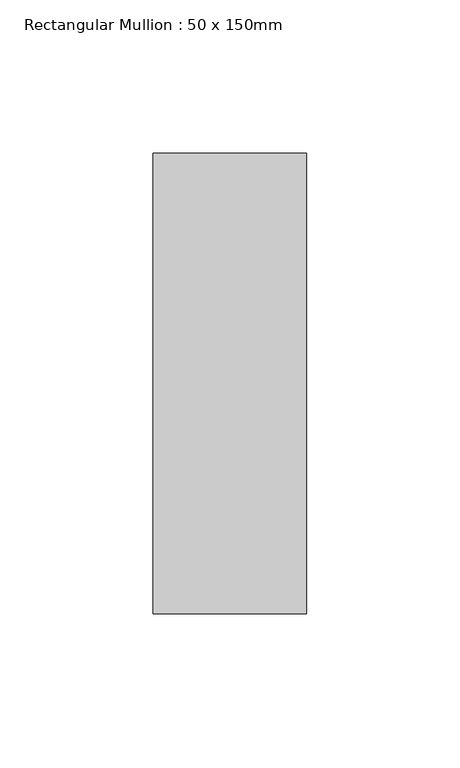
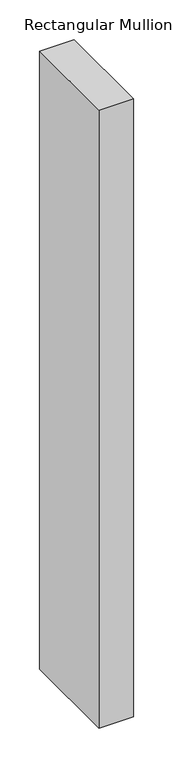
"""IFC4 building model written with IfcOpenShell, lengths in millimetres: member geometry, Rectangular Mullion : 50 x 150mm."""

import ifcopenshell
import ifcopenshell.guid

model = None  # the IFC model being written
_history = None  # IfcOwnerHistory: only IFC2X3 demands one
_inside = {}  # id of a spatial element -> (the spatial element, [elements in it])
_under = {}  # id of a project, library or spatial element -> (it, [spatial elements below it])
_declared = {}  # id of a project -> (the project, [libraries it declares])
_typed = {}  # id of a type object -> (the type object, [elements of that type])
_made_of = {}  # id of a material, layer set ... -> (it, [elements and type objects made of it])


def new_model(schema):
    """Start an empty IFC model of exactly this schema.

    Asked for "IFC4X3", IfcOpenShell would pick the latest addendum, in which some entities
    have other attributes; the version numbers below select the first issue.
    IFC2X3 requires an IfcOwnerHistory on every rooted entity: one is made here for all.
    """
    global model, _history
    if schema == "IFC4X3":
        model = ifcopenshell.file(schema_version=(4, 3, 0, 0))
    else:
        model = ifcopenshell.file(schema=schema)
    _inside.clear()
    _under.clear()
    _declared.clear()
    _typed.clear()
    _made_of.clear()
    _history = None
    if model.schema == "IFC2X3":
        org = make("IfcOrganization", Name="unknown")
        user = make(
            "IfcPersonAndOrganization",
            ThePerson=make("IfcPerson", FamilyName="unknown"),
            TheOrganization=org,
        )
        app = make(
            "IfcApplication",
            ApplicationDeveloper=org,
            Version="unknown",
            ApplicationFullName="unknown",
            ApplicationIdentifier="unknown",
        )
        _history = make(
            "IfcOwnerHistory",
            OwningUser=user,
            OwningApplication=app,
            ChangeAction="ADDED",
            CreationDate=0,
        )
    return model


def make(cls, **values):
    """One entity of the class cls with the attributes given. An attribute that is None is left unset."""
    return model.create_entity(
        cls, **{name: value for name, value in values.items() if value is not None}
    )


def rooted(cls, **values):
    """An entity with a GlobalId (a new one), such as an element, a storey or a relation."""
    return make(cls, GlobalId=ifcopenshell.guid.new(), OwnerHistory=_history, **values)


def si_unit(unit_type, name, prefix=None):
    """IfcSIUnit, for example si_unit("LENGTHUNIT", "METRE", prefix="MILLI")."""
    return make("IfcSIUnit", UnitType=unit_type, Prefix=prefix, Name=name)


def assignment(units):
    """IfcUnitAssignment: the units of a project."""
    return None if units is None else make("IfcUnitAssignment", Units=units)


def point(xyz):
    """IfcCartesianPoint."""
    return None if xyz is None else make("IfcCartesianPoint", Coordinates=xyz)


def direction(xyz):
    """IfcDirection."""
    return None if xyz is None else make("IfcDirection", DirectionRatios=xyz)


def frame(location, z_axis=None, x_axis=None):
    """IfcAxis2Placement3D, a coordinate frame: its origin and axes. An axis left out is left unset."""
    return make(
        "IfcAxis2Placement3D",
        Location=point(location),
        Axis=direction(z_axis),
        RefDirection=direction(x_axis),
    )


def origin():
    """The frame at (0, 0, 0) with its axes left unset."""
    return frame((0.0, 0.0, 0.0))


def place(relative_to, where):
    """IfcLocalPlacement: puts the frame where relative to a parent placement (None: the world)."""
    return make(
        "IfcLocalPlacement", PlacementRelTo=relative_to, RelativePlacement=where
    )


def context(
    kind, dimensions, precision=None, world=None, true_north=None, identifier=None
):
    """IfcGeometricRepresentationContext, for example the 3D "Model" context."""
    return make(
        "IfcGeometricRepresentationContext",
        ContextIdentifier=identifier,
        ContextType=kind,
        CoordinateSpaceDimension=dimensions,
        Precision=precision,
        WorldCoordinateSystem=world,
        TrueNorth=true_north,
    )


def project(units=None, contexts=None):
    """IfcProject with its units and contexts."""
    return rooted(
        "IfcProject",
        Name="project",
        RepresentationContexts=contexts,
        UnitsInContext=assignment(units),
    )


def spatial(cls, under=None, at=None, **own):
    """A site, building, storey or space (cls), placed at a placement, below another one or the project."""
    s = rooted(cls, ObjectPlacement=at, **own)
    if under is not None:
        _under.setdefault(under.id(), (under, []))[1].append(s)
    return s


def polyline(points):
    """IfcPolyline through the points."""
    return make("IfcPolyline", Points=[point(p) for p in points])


def outline(outer, holes=None, kind="AREA"):
    """IfcArbitraryClosedProfileDef: a profile drawn as a closed curve; with holes, ...WithVoids."""
    if holes is None:
        return make("IfcArbitraryClosedProfileDef", ProfileType=kind, OuterCurve=outer)
    return make(
        "IfcArbitraryProfileDefWithVoids",
        ProfileType=kind,
        OuterCurve=outer,
        InnerCurves=holes,
    )


def extrude(swept, where, along, depth):
    """IfcExtrudedAreaSolid: the profile swept, set in the frame where, extruded along a direction by depth."""
    return make(
        "IfcExtrudedAreaSolid",
        SweptArea=swept,
        Position=where,
        ExtrudedDirection=direction(along),
        Depth=depth,
    )


def shape(context_of_items, identifier, shape_type, items):
    """IfcShapeRepresentation: the items that make up one representation, for example the "Body"."""
    return make(
        "IfcShapeRepresentation",
        ContextOfItems=context_of_items,
        RepresentationIdentifier=identifier,
        RepresentationType=shape_type,
        Items=items,
    )


def source(mapping_origin, context_of_items, identifier, shape_type, items):
    """IfcRepresentationMap: a shape defined once, which mapped items show again and again."""
    return make(
        "IfcRepresentationMap",
        MappingOrigin=mapping_origin,
        MappedRepresentation=shape(context_of_items, identifier, shape_type, items),
    )


def transform(
    local_origin,
    x_axis=None,
    y_axis=None,
    z_axis=None,
    scale=None,
    scale2=None,
    scale3=None,
    uniform=True,
):
    """IfcCartesianTransformationOperator3D, or its non-uniform kind. x_axis, y_axis, z_axis: its Axis1, 2, 3."""
    if uniform:
        return make(
            "IfcCartesianTransformationOperator3D",
            Axis1=direction(x_axis),
            Axis2=direction(y_axis),
            LocalOrigin=point(local_origin),
            Scale=scale,
            Axis3=direction(z_axis),
        )
    return make(
        "IfcCartesianTransformationOperator3DnonUniform",
        Axis1=direction(x_axis),
        Axis2=direction(y_axis),
        LocalOrigin=point(local_origin),
        Scale=scale,
        Axis3=direction(z_axis),
        Scale2=scale2,
        Scale3=scale3,
    )


def mapped(mapping_source, mapping_target):
    """IfcMappedItem: shows the shape of a source again, moved by a transform."""
    return make(
        "IfcMappedItem", MappingSource=mapping_source, MappingTarget=mapping_target
    )


def made_of(thing, what):
    """Note that an element or type object is made of a material, layer set ...; save() writes the relation."""
    if what is not None:
        _made_of.setdefault(what.id(), (what, []))[1].append(thing)
    return thing


def element(
    cls,
    number,
    at=None,
    inside=None,
    cuts=None,
    type_object=None,
    material=None,
    context=None,
    identifier="Body",
    shape_type=None,
    held_by="IfcProductDefinitionShape",
    body=None,
    shapes=None,
    **own,
):
    """One element of the class cls, such as IfcWall. Its Tag is "e" and its number.

    at: its placement. inside: the storey or other place that contains it. cuts: it is an
    opening in that element (IfcRelVoidsElement). A single representation is given by context,
    identifier, shape_type and body (its items); several are given by shapes. held_by: the class
    of the entity that holds the representations. save() writes the other relations.
    """
    e = rooted(cls, Tag="e%d" % number, ObjectPlacement=at, **own)
    if body is not None:
        shapes = [shape(context, identifier, shape_type, body)]
    if shapes is not None:
        e.Representation = make(held_by, Representations=shapes)
    if inside is not None:
        _inside.setdefault(inside.id(), (inside, []))[1].append(e)
    if cuts is not None:
        rooted(
            "IfcRelVoidsElement", RelatingBuildingElement=cuts, RelatedOpeningElement=e
        )
    if type_object is not None:
        _typed.setdefault(type_object.id(), (type_object, []))[1].append(e)
    return made_of(e, material)


def aggregate(whole, parts):
    """IfcRelAggregates: a whole, such as a stair, and the parts it consists of."""
    return rooted("IfcRelAggregates", RelatingObject=whole, RelatedObjects=parts)


def save(model, path):
    """Write the relations noted so far, then the file.

    IfcRelAggregates (storeys below a building ...), IfcRelContainedInSpatialStructure (elements
    in a storey), IfcRelDefinesByType, IfcRelAssociatesMaterial and IfcRelDeclares: one each for
    every whole, place, type object, material and project.
    """
    for whole, parts in _under.values():
        aggregate(whole, parts)
    for where, things in _inside.values():
        rooted(
            "IfcRelContainedInSpatialStructure",
            RelatedElements=things,
            RelatingStructure=where,
        )
    for kind, things in _typed.values():
        rooted("IfcRelDefinesByType", RelatedObjects=things, RelatingType=kind)
    for what, things in _made_of.values():
        rooted("IfcRelAssociatesMaterial", RelatedObjects=things, RelatingMaterial=what)
    for by, libraries in _declared.values():
        rooted("IfcRelDeclares", RelatingContext=by, RelatedDefinitions=libraries)
    model.write(path)


def rectangular_mullion_50_x_150mm_a053b0ca(model_context):
    return source(origin(), model_context, "Body", "SweptSolid", [
        extrude(outline(polyline([(25.0, 75.0), (25.0, -75.0), (-25.0, -75.0), (-25.0, 75.0), (25.0, 75.0)])), frame((0.0, 0.0, -950.0), z_axis=(0.0, 0.0, 1.0), x_axis=(1.0, 0.0, 0.0)), (0.0, 0.0, 1.0), 950.0),
    ])


if __name__ == "__main__":
    model = new_model("IFC4")
    model_context = context("Model", 3, world=origin())
    ifc_project = project(units=[si_unit("LENGTHUNIT", "METRE", prefix="MILLI")], contexts=[model_context])
    site = spatial("IfcSite", under=ifc_project)
    building = spatial("IfcBuilding", under=site)
    placement = place(None, origin())
    rectangular_mullion_50_x_150mm_shape = rectangular_mullion_50_x_150mm_a053b0ca(model_context)
    element("IfcMember", 1, ObjectType="Rectangular Mullion : 50 x 150mm", at=placement, inside=building, context=model_context, shape_type="MappedRepresentation", body=[
        mapped(rectangular_mullion_50_x_150mm_shape, transform((0.0, 0.0, 0.0), x_axis=(1.0, 0.0, 0.0), y_axis=(0.0, 1.0, 0.0), z_axis=(0.0, 0.0, 1.0))),
    ])
    save(model, "model.ifc")

# Revit data of these elements
# Type "Rectangular Mullion : 50 x 150mm"
#   built-in parameter 1007304 = 0.492126 (stored number, unit not read)
#   built-in parameter 1007301 = 0.082021 (stored number, unit not read)
#   built-in parameter 1007300 = 0.082021 (stored number, unit not read)
# Element 1 (IfcMember, "Rectangular Mullion : 50 x 150mm")
#   Materials on its faces: "Aluminium"
# Materials
#   "Aluminium": class "Metal", colour RGB 247 247 247, transparency 0, Description = "Aluminium 6061", Cost = 0
